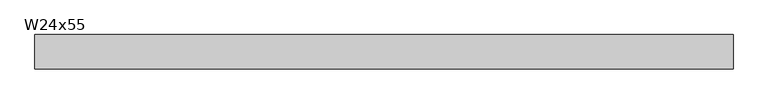
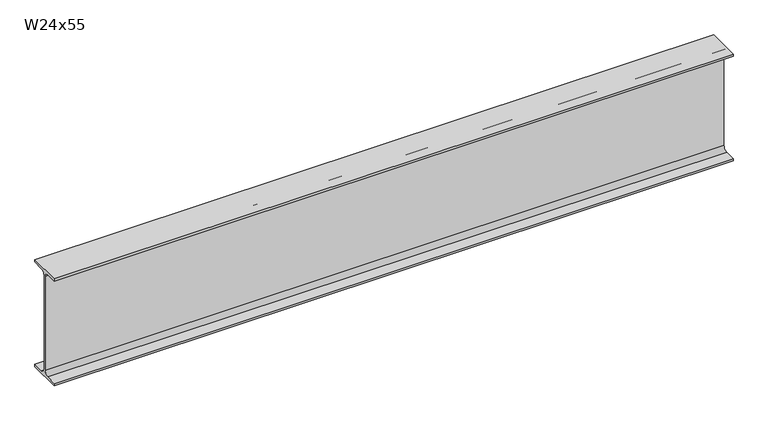
"""IFC4 building model written with IfcOpenShell, lengths in millimetres: beam geometry, RME W-Wide Flange : W24x55."""

from ifc_helpers import new_model, si_unit, point, frame, frame_2d, origin, place, context, project, spatial, polyline, circle_curve, trimmed, segment, composite_curve, outline, extrude, source, transform, mapped, element, save


def w24x55_6716647d(model_context):
    return source(origin(), model_context, "Body", "SweptSolid", [
        extrude(outline(composite_curve([segment(polyline([(89.027, -286.893), (89.027, -299.72), (-89.027, -299.72), (-89.027, -286.893), (-28.702, -286.893)]), True, "CONTINUOUS"), segment(trimmed(circle_curve(frame_2d((-28.702, -263.2075)), 23.6855), [point((-28.702, -286.893))], [point((-5.0165, -263.2075))], True, "CARTESIAN"), True, "CONTINUOUS"), segment(polyline([(-5.0165, -263.2075), (-5.0165, 263.2075)]), True, "CONTINUOUS"), segment(trimmed(circle_curve(frame_2d((-28.702, 263.2075)), 23.6855), [point((-5.0165, 263.2075))], [point((-28.702, 286.893))], True, "CARTESIAN"), True, "CONTINUOUS"), segment(polyline([(-28.702, 286.893), (-89.027, 286.893), (-89.027, 299.72), (89.027, 299.72), (89.027, 286.893), (28.702, 286.893)]), True, "CONTINUOUS"), segment(trimmed(circle_curve(frame_2d((28.702, 263.2075)), 23.6855), [point((28.702, 286.893))], [point((5.0165, 263.2075))], True, "CARTESIAN"), True, "CONTINUOUS"), segment(polyline([(5.0165, 263.2075), (5.0165, -263.2075)]), True, "CONTINUOUS"), segment(trimmed(circle_curve(frame_2d((28.702, -263.2075)), 23.6855), [point((5.0165, -263.2075))], [point((28.702, -286.893))], True, "CARTESIAN"), True, "CONTINUOUS"), segment(polyline([(28.702, -286.893), (89.027, -286.893)]), True, "CONTINUOUS")], self_intersect=False)), frame((-1780.1781867, 0.0, 0.0), z_axis=(1.0, 0.0, 0.0), x_axis=(0.0, 1.0, 0.0)), (0.0, 0.0, 1.0), 3602.3685541),
    ])


if __name__ == "__main__":
    model = new_model("IFC4")
    model_context = context("Model", 3, world=origin())
    ifc_project = project(units=[si_unit("LENGTHUNIT", "METRE", prefix="MILLI")], contexts=[model_context])
    site = spatial("IfcSite", under=ifc_project)
    building = spatial("IfcBuilding", under=site)
    placement = place(None, origin())
    w24x55_shape = w24x55_6716647d(model_context)
    element("IfcBeam", 1, ObjectType="RME W-Wide Flange : W24x55", at=placement, inside=building, context=model_context, shape_type="MappedRepresentation", body=[
        mapped(w24x55_shape, transform((0.0, 0.0, 0.0), x_axis=(1.0, 0.0, 0.0), y_axis=(0.0, 1.0, 0.0), z_axis=(0.0, 0.0, 1.0))),
    ])
    save(model, "model.ifc")

# Revit data of these elements
# Type "RME W-Wide Flange : W24x55"
#   WELD P [instance default] = ""
#   WELD LE [instance default] = ""
#   WELD D [instance default] = ""
#   TOP SECTION SIZE [instance default] = ""
#   TOP SECTION LENGTH [instance default] = ""
#   REMARKS [instance default] = ""
#   REINF TYPE [instance default] = ""
#   Nominal Size = "W24"
#   End Bearing Capacity [instance default] = ""
#   BOT SECTION SIZE [instance default] = ""
#   BOT SECTION LENGTH [instance default] = ""
#   Assembly Code = "B10"
#   W = 55
#   Start Extension Calculation [instance default] = 10' - 0"
#   Start Extension [instance default] = -0' - 0 1/2"
#   End Extension Calculation [instance default] = 10' - 0"
#   End Extension [instance default] = -0' - 0 1/2"
#   Length [instance default] = 5' - 0"
#   bf = 0' - 7.01"
#   d = 1' - 11.6"
#   k = 0' - 1 7/16"
#   k2 = 0' - 0.9325"
#   tf = 0' - 0.505"
#   tw = 0' - 0.395"
#   A = 0.1125 SF
#   Structural Material [instance default] = Metal - Steel - ASTM A992
# Element 1 (IfcBeam, "RME W-Wide Flange : W24x55")
#   Length = 12' - 7.96711"
#   Materials on its faces: "Metal - Steel - ASTM A992"
# Materials
#   "Metal - Steel - ASTM A992": class "Metal", colour RGB 255 128 0, transparency 0
